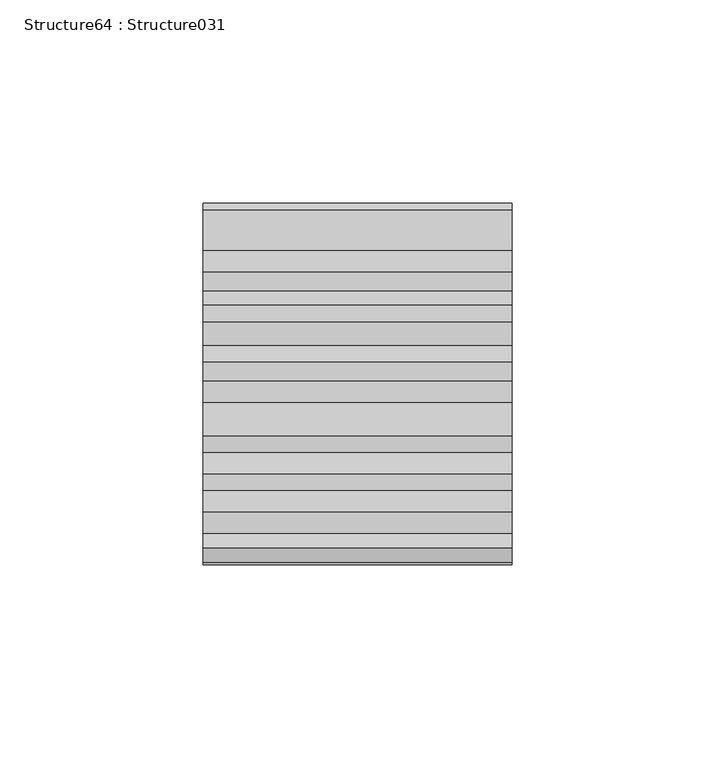
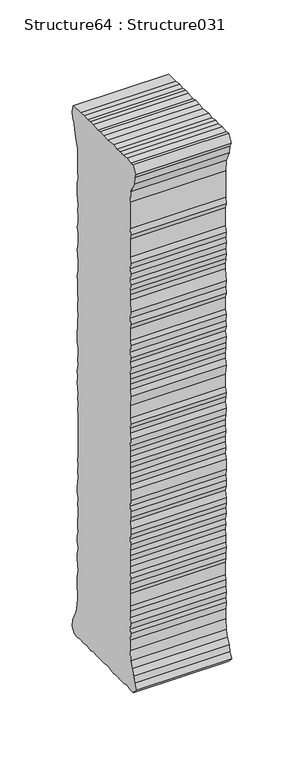
"""IFC4 building model written with IfcOpenShell, lengths in millimetres: proxy geometry, Structure64 : Structure031."""

import ifcopenshell
import ifcopenshell.guid

model = None  # the IFC model being written
_history = None  # IfcOwnerHistory: only IFC2X3 demands one
_inside = {}  # id of a spatial element -> (the spatial element, [elements in it])
_under = {}  # id of a project, library or spatial element -> (it, [spatial elements below it])
_declared = {}  # id of a project -> (the project, [libraries it declares])
_typed = {}  # id of a type object -> (the type object, [elements of that type])
_made_of = {}  # id of a material, layer set ... -> (it, [elements and type objects made of it])


def new_model(schema):
    """Start an empty IFC model of exactly this schema.

    Asked for "IFC4X3", IfcOpenShell would pick the latest addendum, in which some entities
    have other attributes; the version numbers below select the first issue.
    IFC2X3 requires an IfcOwnerHistory on every rooted entity: one is made here for all.
    """
    global model, _history
    if schema == "IFC4X3":
        model = ifcopenshell.file(schema_version=(4, 3, 0, 0))
    else:
        model = ifcopenshell.file(schema=schema)
    _inside.clear()
    _under.clear()
    _declared.clear()
    _typed.clear()
    _made_of.clear()
    _history = None
    if model.schema == "IFC2X3":
        org = make("IfcOrganization", Name="unknown")
        user = make(
            "IfcPersonAndOrganization",
            ThePerson=make("IfcPerson", FamilyName="unknown"),
            TheOrganization=org,
        )
        app = make(
            "IfcApplication",
            ApplicationDeveloper=org,
            Version="unknown",
            ApplicationFullName="unknown",
            ApplicationIdentifier="unknown",
        )
        _history = make(
            "IfcOwnerHistory",
            OwningUser=user,
            OwningApplication=app,
            ChangeAction="ADDED",
            CreationDate=0,
        )
    return model


def make(cls, **values):
    """One entity of the class cls with the attributes given. An attribute that is None is left unset."""
    return model.create_entity(
        cls, **{name: value for name, value in values.items() if value is not None}
    )


def rooted(cls, **values):
    """An entity with a GlobalId (a new one), such as an element, a storey or a relation."""
    return make(cls, GlobalId=ifcopenshell.guid.new(), OwnerHistory=_history, **values)


def si_unit(unit_type, name, prefix=None):
    """IfcSIUnit, for example si_unit("LENGTHUNIT", "METRE", prefix="MILLI")."""
    return make("IfcSIUnit", UnitType=unit_type, Prefix=prefix, Name=name)


def assignment(units):
    """IfcUnitAssignment: the units of a project."""
    return None if units is None else make("IfcUnitAssignment", Units=units)


def point(xyz):
    """IfcCartesianPoint."""
    return None if xyz is None else make("IfcCartesianPoint", Coordinates=xyz)


def direction(xyz):
    """IfcDirection."""
    return None if xyz is None else make("IfcDirection", DirectionRatios=xyz)


def frame(location, z_axis=None, x_axis=None):
    """IfcAxis2Placement3D, a coordinate frame: its origin and axes. An axis left out is left unset."""
    return make(
        "IfcAxis2Placement3D",
        Location=point(location),
        Axis=direction(z_axis),
        RefDirection=direction(x_axis),
    )


def origin():
    """The frame at (0, 0, 0) with its axes left unset."""
    return frame((0.0, 0.0, 0.0))


def place(relative_to, where):
    """IfcLocalPlacement: puts the frame where relative to a parent placement (None: the world)."""
    return make(
        "IfcLocalPlacement", PlacementRelTo=relative_to, RelativePlacement=where
    )


def context(
    kind, dimensions, precision=None, world=None, true_north=None, identifier=None
):
    """IfcGeometricRepresentationContext, for example the 3D "Model" context."""
    return make(
        "IfcGeometricRepresentationContext",
        ContextIdentifier=identifier,
        ContextType=kind,
        CoordinateSpaceDimension=dimensions,
        Precision=precision,
        WorldCoordinateSystem=world,
        TrueNorth=true_north,
    )


def project(units=None, contexts=None):
    """IfcProject with its units and contexts."""
    return rooted(
        "IfcProject",
        Name="project",
        RepresentationContexts=contexts,
        UnitsInContext=assignment(units),
    )


def spatial(cls, under=None, at=None, **own):
    """A site, building, storey or space (cls), placed at a placement, below another one or the project."""
    s = rooted(cls, ObjectPlacement=at, **own)
    if under is not None:
        _under.setdefault(under.id(), (under, []))[1].append(s)
    return s


def polyline(points):
    """IfcPolyline through the points."""
    return make("IfcPolyline", Points=[point(p) for p in points])


def outline(outer, holes=None, kind="AREA"):
    """IfcArbitraryClosedProfileDef: a profile drawn as a closed curve; with holes, ...WithVoids."""
    if holes is None:
        return make("IfcArbitraryClosedProfileDef", ProfileType=kind, OuterCurve=outer)
    return make(
        "IfcArbitraryProfileDefWithVoids",
        ProfileType=kind,
        OuterCurve=outer,
        InnerCurves=holes,
    )


def extrude(swept, where, along, depth):
    """IfcExtrudedAreaSolid: the profile swept, set in the frame where, extruded along a direction by depth."""
    return make(
        "IfcExtrudedAreaSolid",
        SweptArea=swept,
        Position=where,
        ExtrudedDirection=direction(along),
        Depth=depth,
    )


def shape(context_of_items, identifier, shape_type, items):
    """IfcShapeRepresentation: the items that make up one representation, for example the "Body"."""
    return make(
        "IfcShapeRepresentation",
        ContextOfItems=context_of_items,
        RepresentationIdentifier=identifier,
        RepresentationType=shape_type,
        Items=items,
    )


def source(mapping_origin, context_of_items, identifier, shape_type, items):
    """IfcRepresentationMap: a shape defined once, which mapped items show again and again."""
    return make(
        "IfcRepresentationMap",
        MappingOrigin=mapping_origin,
        MappedRepresentation=shape(context_of_items, identifier, shape_type, items),
    )


def transform(
    local_origin,
    x_axis=None,
    y_axis=None,
    z_axis=None,
    scale=None,
    scale2=None,
    scale3=None,
    uniform=True,
):
    """IfcCartesianTransformationOperator3D, or its non-uniform kind. x_axis, y_axis, z_axis: its Axis1, 2, 3."""
    if uniform:
        return make(
            "IfcCartesianTransformationOperator3D",
            Axis1=direction(x_axis),
            Axis2=direction(y_axis),
            LocalOrigin=point(local_origin),
            Scale=scale,
            Axis3=direction(z_axis),
        )
    return make(
        "IfcCartesianTransformationOperator3DnonUniform",
        Axis1=direction(x_axis),
        Axis2=direction(y_axis),
        LocalOrigin=point(local_origin),
        Scale=scale,
        Axis3=direction(z_axis),
        Scale2=scale2,
        Scale3=scale3,
    )


def mapped(mapping_source, mapping_target):
    """IfcMappedItem: shows the shape of a source again, moved by a transform."""
    return make(
        "IfcMappedItem", MappingSource=mapping_source, MappingTarget=mapping_target
    )


def made_of(thing, what):
    """Note that an element or type object is made of a material, layer set ...; save() writes the relation."""
    if what is not None:
        _made_of.setdefault(what.id(), (what, []))[1].append(thing)
    return thing


def element(
    cls,
    number,
    at=None,
    inside=None,
    cuts=None,
    type_object=None,
    material=None,
    context=None,
    identifier="Body",
    shape_type=None,
    held_by="IfcProductDefinitionShape",
    body=None,
    shapes=None,
    **own,
):
    """One element of the class cls, such as IfcWall. Its Tag is "e" and its number.

    at: its placement. inside: the storey or other place that contains it. cuts: it is an
    opening in that element (IfcRelVoidsElement). A single representation is given by context,
    identifier, shape_type and body (its items); several are given by shapes. held_by: the class
    of the entity that holds the representations. save() writes the other relations.
    """
    e = rooted(cls, Tag="e%d" % number, ObjectPlacement=at, **own)
    if body is not None:
        shapes = [shape(context, identifier, shape_type, body)]
    if shapes is not None:
        e.Representation = make(held_by, Representations=shapes)
    if inside is not None:
        _inside.setdefault(inside.id(), (inside, []))[1].append(e)
    if cuts is not None:
        rooted(
            "IfcRelVoidsElement", RelatingBuildingElement=cuts, RelatedOpeningElement=e
        )
    if type_object is not None:
        _typed.setdefault(type_object.id(), (type_object, []))[1].append(e)
    return made_of(e, material)


def aggregate(whole, parts):
    """IfcRelAggregates: a whole, such as a stair, and the parts it consists of."""
    return rooted("IfcRelAggregates", RelatingObject=whole, RelatedObjects=parts)


def save(model, path):
    """Write the relations noted so far, then the file.

    IfcRelAggregates (storeys below a building ...), IfcRelContainedInSpatialStructure (elements
    in a storey), IfcRelDefinesByType, IfcRelAssociatesMaterial and IfcRelDeclares: one each for
    every whole, place, type object, material and project.
    """
    for whole, parts in _under.values():
        aggregate(whole, parts)
    for where, things in _inside.values():
        rooted(
            "IfcRelContainedInSpatialStructure",
            RelatedElements=things,
            RelatingStructure=where,
        )
    for kind, things in _typed.values():
        rooted("IfcRelDefinesByType", RelatedObjects=things, RelatingType=kind)
    for what, things in _made_of.values():
        rooted("IfcRelAssociatesMaterial", RelatedObjects=things, RelatingMaterial=what)
    for by, libraries in _declared.values():
        rooted("IfcRelDeclares", RelatingContext=by, RelatedDefinitions=libraries)
    model.write(path)


def structure64_structure031_c65267a2(model_context):
    return source(origin(), model_context, "Body", "SweptSolid", [
        extrude(outline(polyline([(281027.8807777, 3575.6853037), (281028.4632491, 3583.8864372), (281028.4632491, 3592.6700423), (281027.8807777, 3598.5284533), (281028.4632491, 3602.0280957), (281027.8807777, 3606.7295868), (281028.4632491, 3611.4134274), (281028.4632491, 3617.2718384), (281029.0553481, 3620.7971545), (281029.0553481, 3631.3410106), (281028.4632491, 3634.856699), (281028.4632491, 3640.114988), (281027.8807777, 3644.8245022), (281028.4632491, 3648.9258713), (281028.4632491, 3654.7842823), (281029.0553481, 3659.4584952), (281028.4632491, 3664.1423357), (281029.0553481, 3668.2437048), (281027.8807777, 3673.5276674), (281028.4632491, 3678.2018803), (281027.8807777, 3682.3289231), (281027.8807777, 3687.0127636), (281029.0553481, 3692.2710525), (281027.8807777, 3696.3884676), (281027.8807777, 3701.6547796), (281028.4632491, 3705.7545441), (281027.8807777, 3711.0304837), (281027.8807777, 3719.2316172), (281029.0553481, 3723.9154578), (281028.4632491, 3728.5992983), (281029.0553481, 3733.2991849), (281029.0553481, 3737.9750024), (281028.4632491, 3742.6748889), (281029.0553481, 3747.3587295), (281029.0553481, 3752.04257), (281028.4632491, 3756.7440611), (281027.8807777, 3762.5848215), (281029.0553481, 3767.2590344), (281028.4632491, 3771.9605256), (281027.8807777, 3775.4874463), (281029.0553481, 3780.1616592), (281029.0553481, 3790.7039107), (281027.8807777, 3798.9050443), (281029.0553481, 3804.1890069), (281029.0553481, 3808.8888934), (281028.4632491, 3813.5743386), (281028.4632491, 3817.6741031), (281027.8807777, 3822.932392), (281029.0553481, 3827.6162325), (281027.8807777, 3831.732043), (281028.4632491, 3836.4174882), (281027.8807777, 3842.2758992), (281029.0553481, 3845.8012153), (281029.0553481, 3855.7353217), (281027.8807777, 3859.8591552), (281028.4632491, 3865.1190488), (281027.8807777, 3870.4030114), (281029.0553481, 3879.7610648), (281029.0553481, 3884.4609514), (281028.4632491, 3888.5623205), (281027.8807777, 3893.246161), (281028.4632491, 3897.3475301), (281027.8807777, 3902.6314927), (281028.4632491, 3906.7328618), (281027.8807777, 3911.4054701), (281029.0553481, 3916.0909152), (281029.0553481, 3931.3346579), (281027.8807777, 3935.4328178), (281028.4632491, 3940.718385), (281028.4632491, 3962.9774586), (281027.8807777, 3972.3627903), (281023.1969371, 3981.7208437), (281022.6128611, 3987.5792547), (281020.8445869, 3991.0788971), (281024.3634846, 3997.5486624), (281027.8807777, 3996.390138), (281033.1567172, 3997.5486624), (281038.4230292, 3996.9645864), (281042.5324213, 3997.5486624), (281047.8067563, 3996.390138), (281051.9081254, 3997.5486624), (281060.117282, 3996.390138), (281065.3835939, 3996.9645864), (281070.0658298, 3997.5486624), (281074.1671989, 3996.390138), (281080.02561, 3997.5486624), (281084.126979, 3997.5486624), (281087.6442721, 3996.9645864), (281092.3377402, 3997.5486624), (281097.6120752, 3996.9645864), (281107.5702507, 3996.9645864), (281109.3305019, 3991.0788971), (281108.1543268, 3986.4046842), (281106.3956802, 3982.3225704), (281105.8051858, 3978.2035506), (281104.0529577, 3972.3627903), (281101.7134443, 3964.1343784), (281101.7134443, 3944.8165449), (281101.1293683, 3939.5325823), (281102.2862881, 3935.4328178), (281102.2862881, 3925.4746423), (281101.7134443, 3921.3748778), (281101.1293683, 3916.6653636), (281101.7134443, 3911.4054701), (281101.1293683, 3907.888177), (281101.1293683, 3903.2059411), (281102.2862881, 3897.3475301), (281101.1293683, 3893.246161), (281101.1293683, 3883.8881076), (281102.2862881, 3878.5784713), (281101.7134443, 3874.5043805), (281101.1293683, 3869.2444869), (281101.1293683, 3861.0192843), (281102.2862881, 3856.3161885), (281101.7134443, 3851.6612309), (281101.7134443, 3841.0900965), (281101.1293683, 3836.9919366), (281101.7134443, 3832.8921721), (281101.7134443, 3828.2163546), (281101.1293683, 3822.932392), (281101.7134443, 3818.8310229), (281101.7134443, 3812.9726119), (281102.2862881, 3808.8888934), (281102.2862881, 3800.0876378), (281101.1293683, 3795.4037973), (281101.1293683, 3790.7039107), (281101.7134443, 3785.4456218), (281101.1293683, 3781.3282066), (281102.2862881, 3776.0618947), (281101.7134443, 3770.8036057), (281102.2862881, 3766.1021146), (281101.7134443, 3762.0023501), (281101.1293683, 3756.7440611), (281101.7134443, 3753.2171405), (281101.1293683, 3748.5429276), (281101.7134443, 3742.6748889), (281101.1293683, 3739.1592005), (281101.1293683, 3705.7545441), (281101.7134443, 3700.4705815), (281101.1293683, 3696.3884676), (281101.7134443, 3691.0868544), (281101.1293683, 3686.4030139), (281101.7134443, 3681.7271964), (281102.2862881, 3677.6274319), (281102.2862881, 3673.5276674), (281101.1293683, 3668.8261762), (281101.7134443, 3663.5598643), (281101.1293683, 3658.8840468), (281101.1293683, 3654.1841602), (281101.7134443, 3649.5003197), (281101.7134443, 3644.2420307), (281101.1293683, 3640.114988), (281102.2862881, 3636.0408972), (281102.2862881, 3631.3410106), (281101.1293683, 3626.6571701), (281102.2862881, 3620.7971545), (281102.2862881, 3616.69739), (281101.7134443, 3612.5976255), (281101.1293683, 3607.3393366), (281102.2862881, 3602.0280957), (281102.2862881, 3592.6700423), (281101.7134443, 3587.9685511), (281101.7134443, 3583.2863152), (281102.8783872, 3573.9266571), (281104.6370337, 3569.8268927), (281106.3956802, 3565.7094775), (281108.7464258, 3561.025637), (281109.3305019, 3555.1848766), (281106.3956802, 3551.0658569), (281102.8783872, 3550.4833855), (281098.1945467, 3551.0658569), (281092.3377402, 3551.0658569), (281088.8188426, 3551.6675836), (281083.542903, 3550.4833855), (281080.02561, 3551.6675836), (281075.3497925, 3551.0658569), (281064.7914949, 3551.0658569), (281060.117282, 3551.6675836), (281056.0078899, 3551.0658569), (281051.3144217, 3550.4833855), (281047.2146572, 3551.0658569), (281042.5324213, 3550.4833855), (281037.2661094, 3550.4833855), (281033.7472117, 3551.6675836), (281028.4632491, 3550.4833855), (281024.3634846, 3550.4833855), (281020.2637201, 3555.1848766), (281022.6128611, 3559.8671125), (281023.7810132, 3565.1254015), (281026.1317588, 3569.8268927), (281027.8807777, 3575.6853037)])), frame((-59031.6926606, 0.0, 0.0), z_axis=(1.0, 0.0, 0.0), x_axis=(0.0, 1.0, 0.0)), (0.0, 0.0, 1.0), 76.2),
    ])


if __name__ == "__main__":
    model = new_model("IFC4")
    model_context = context("Model", 3, world=origin())
    ifc_project = project(units=[si_unit("LENGTHUNIT", "METRE", prefix="MILLI")], contexts=[model_context])
    site = spatial("IfcSite", under=ifc_project)
    building = spatial("IfcBuilding", under=site)
    placement = place(None, origin())
    structure64_structure031_shape = structure64_structure031_c65267a2(model_context)
    element("IfcBuildingElementProxy", 1, Name="Structure64 : Structure031", ObjectType="Structure64 : Structure031", at=placement, inside=building, context=model_context, shape_type="MappedRepresentation", body=[
        mapped(structure64_structure031_shape, transform((0.0, 0.0, 0.0), x_axis=(1.0, 0.0, 0.0), y_axis=(0.0, 1.0, 0.0), z_axis=(0.0, 0.0, 1.0))),
    ])
    save(model, "model.ifc")

# Revit data of these elements
# Type "Structure64 : Structure031"
#   NameOverride = "Structure031"
# Element 1 (IfcBuildingElementProxy, "Structure64 : Structure031")
#   Materials on its faces: "BRUSHED ALUM. LETTERING"
# Materials
#   "BRUSHED ALUM. LETTERING": class "Unassigned", colour RGB 169 181 186, transparency 0, Cost = 0
